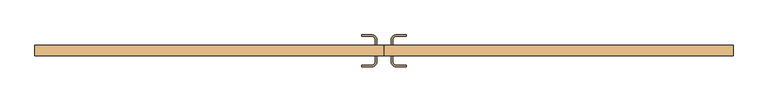
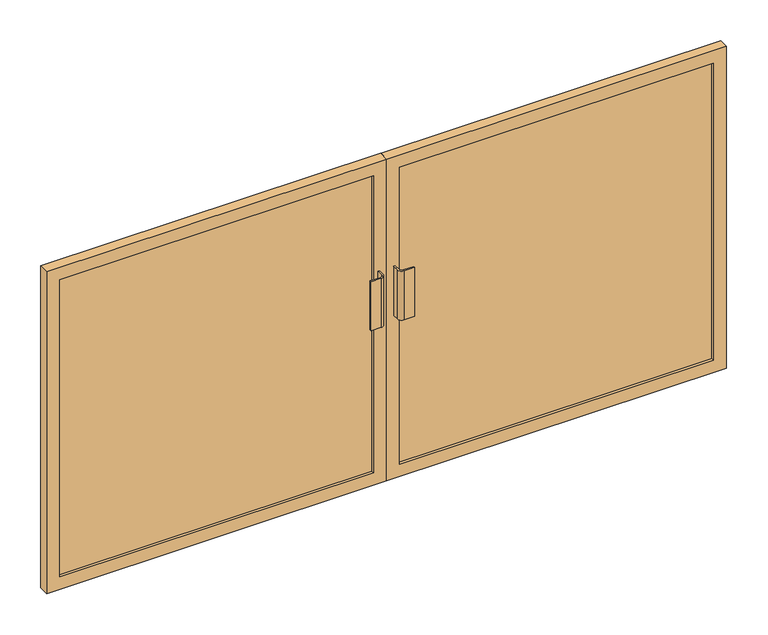
"""IFC4 building model written with IfcOpenShell, lengths in millimetres: door geometry, Porta-Parede-Cortina-Frente de loja-Dupla : Porta-Parede-Cortina-Frente de loja-Dupla."""

from ifc_helpers import new_model, si_unit, point, frame, frame_2d, origin, place, context, project, spatial, polyline, circle_curve, trimmed, segment, composite_curve, outline, extrude, source, transform, mapped, element, save


def door_319e0233(model_context):
    return source(origin(), model_context, "Body", "SweptSolid", [
        extrude(outline(polyline([(1500.0, 0.8168501), (0.0, 0.8168501), (0.0, 1500.0000075), (1500.0, 1500.0000075), (1500.0, 0.8168501)]), holes=[polyline([(1442.85, 57.9668501), (1442.85, 1442.8500075), (57.15, 1442.8500075), (57.15, 57.9668501), (1442.85, 57.9668501)])]), frame((0.0, 15.55, 0.0), z_axis=(0.0, 1.0, 0.0), x_axis=(0.0, 0.0, 1.0)), (0.0, 0.0, 1.0), 44.45),
        extrude(outline(polyline([(1500.0, -0.7706499), (1500.0, -1500.0000075), (0.0, -1500.0000075), (0.0, -0.7706499), (1500.0, -0.7706499)]), holes=[polyline([(1442.85, -1442.8500075), (1442.85, -57.9206499), (57.15, -57.9206499), (57.15, -1442.8500075), (1442.85, -1442.8500075)])]), frame((0.0, 15.55, 0.0), z_axis=(0.0, 1.0, 0.0), x_axis=(0.0, 0.0, 1.0)), (0.0, 0.0, 1.0), 44.45),
        extrude(outline(polyline([(1442.8500075, 28.25), (57.9668501, 28.25), (57.9668501, 47.3), (1442.8500075, 47.3), (1442.8500075, 28.25)])), frame((0.0, 0.0, 57.15), z_axis=(0.0, 0.0, 1.0), x_axis=(1.0, 0.0, 0.0)), (0.0, 0.0, 1.0), 1385.7),
        extrude(outline(polyline([(-57.9206499, 28.25), (-1442.8500075, 28.25), (-1442.8500075, 47.3), (-57.9206499, 47.3), (-57.9206499, 28.25)])), frame((0.0, 0.0, 57.15), z_axis=(0.0, 0.0, 1.0), x_axis=(1.0, 0.0, 0.0)), (0.0, 0.0, 1.0), 1385.7),
        extrude(outline(composite_curve([segment(trimmed(circle_curve(frame_2d((-50.7768999, -12.7)), 19.05), [point((-31.7268999, -12.7))], [point((-50.7768999, -31.75))], False, "CARTESIAN"), True, "CONTINUOUS"), segment(polyline([(-50.7768999, -31.75), (-95.2268999, -31.75), (-95.2268999, -25.4), (-50.7768999, -25.4)]), True, "CONTINUOUS"), segment(trimmed(circle_curve(frame_2d((-50.7768999, -12.7)), 12.7), [point((-50.7768999, -25.4))], [point((-38.0768999, -12.7))], True, "CARTESIAN"), True, "CONTINUOUS"), segment(polyline([(-38.0768999, -12.7), (-38.0768999, 15.55), (-31.7268999, 15.55), (-31.7268999, -12.7)]), True, "CONTINUOUS")], self_intersect=False)), frame((0.0, 0.0, 762.0), z_axis=(0.0, 0.0, 1.0), x_axis=(1.0, 0.0, 0.0)), (0.0, 0.0, 1.0), 228.6),
        extrude(outline(composite_curve([segment(polyline([(31.7731001, -12.7), (31.7731001, 15.55), (38.1231001, 15.55), (38.1231001, -12.7)]), True, "CONTINUOUS"), segment(trimmed(circle_curve(frame_2d((50.8231001, -12.7)), 12.7), [point((38.1231001, -12.7))], [point((50.8231001, -25.4))], True, "CARTESIAN"), True, "CONTINUOUS"), segment(polyline([(50.8231001, -25.4), (95.2731001, -25.4), (95.2731001, -31.75), (50.8231001, -31.75)]), True, "CONTINUOUS"), segment(trimmed(circle_curve(frame_2d((50.8231001, -12.7)), 19.05), [point((50.8231001, -31.75))], [point((31.7731001, -12.7))], False, "CARTESIAN"), True, "CONTINUOUS")], self_intersect=False)), frame((0.0, 0.0, 762.0), z_axis=(0.0, 0.0, 1.0), x_axis=(1.0, 0.0, 0.0)), (0.0, 0.0, 1.0), 228.6),
        extrude(outline(composite_curve([segment(polyline([(-31.7268999, 85.4), (-31.7268999, 60.0), (-38.0768999, 60.0), (-38.0768999, 85.4)]), True, "CONTINUOUS"), segment(trimmed(circle_curve(frame_2d((-50.7768999, 85.4)), 12.7), [point((-38.0768999, 85.4))], [point((-50.7768999, 98.1))], True, "CARTESIAN"), True, "CONTINUOUS"), segment(polyline([(-50.7768999, 98.1), (-95.2268999, 98.1), (-95.2268999, 104.45), (-50.7768999, 104.45)]), True, "CONTINUOUS"), segment(trimmed(circle_curve(frame_2d((-50.7768999, 85.4)), 19.05), [point((-50.7768999, 104.45))], [point((-31.7268999, 85.4))], False, "CARTESIAN"), True, "CONTINUOUS")], self_intersect=False)), frame((0.0, 0.0, 762.0), z_axis=(0.0, 0.0, 1.0), x_axis=(1.0, 0.0, 0.0)), (0.0, 0.0, 1.0), 228.6),
        extrude(outline(composite_curve([segment(trimmed(circle_curve(frame_2d((50.8231001, 85.4)), 19.05), [point((31.7731001, 85.4))], [point((50.8231001, 104.45))], False, "CARTESIAN"), True, "CONTINUOUS"), segment(polyline([(50.8231001, 104.45), (95.2731001, 104.45), (95.2731001, 98.1), (50.8231001, 98.1)]), True, "CONTINUOUS"), segment(trimmed(circle_curve(frame_2d((50.8231001, 85.4)), 12.7), [point((50.8231001, 98.1))], [point((38.1231001, 85.4))], True, "CARTESIAN"), True, "CONTINUOUS"), segment(polyline([(38.1231001, 85.4), (38.1231001, 60.0), (31.7731001, 60.0), (31.7731001, 85.4)]), True, "CONTINUOUS")], self_intersect=False)), frame((0.0, 0.0, 762.0), z_axis=(0.0, 0.0, 1.0), x_axis=(1.0, 0.0, 0.0)), (0.0, 0.0, 1.0), 228.6),
    ])


if __name__ == "__main__":
    model = new_model("IFC4")
    model_context = context("Model", 3, world=origin())
    ifc_project = project(units=[si_unit("LENGTHUNIT", "METRE", prefix="MILLI")], contexts=[model_context])
    site = spatial("IfcSite", under=ifc_project)
    building = spatial("IfcBuilding", under=site)
    placement = place(None, origin())
    door_shape = door_319e0233(model_context)
    element("IfcDoor", 1, ObjectType="Porta-Parede-Cortina-Frente de loja-Dupla : Porta-Parede-Cortina-Frente de loja-Dupla", at=placement, inside=building, context=model_context, shape_type="MappedRepresentation", body=[
        mapped(door_shape, transform((0.0, 0.0, 0.0), x_axis=(1.0, 0.0, 0.0), y_axis=(0.0, 1.0, 0.0), z_axis=(0.0, 0.0, 1.0))),
    ])
    save(model, "model.ifc")

# Revit data of these elements
# Type "Porta-Parede-Cortina-Frente de loja-Dupla : Porta-Parede-Cortina-Frente de loja-Dupla"
#   Type Mark = "40"
#   Construction Type Id = "opn-d46"
#   Assembly Code = "B2030100"
#   Analytic Construction = "Moldura de metal, porta de vidro duplo"
#   Largura [instance default] = 1.80 m
#   Thermal Resistance (R) = 0.242926 (m²·K)/W
#   Ângulo de abertura [instance default] = 90.00°
#   Largura do painel [instance default] = 0.90 m
#   Deslocamento = 0.06 m
#   Heat Transfer Coefficient (U) = 4.11674 W/(m²·K)
#   Function = 1
#   Material da moldura = Alumín. 1
#   Material da maçaneta = Alumín. 1
#   Vidraça = Vidro
#   Visual Light Transmittance = 0
#   Solar Heat Gain Coefficient = 0
# Element 1 (IfcDoor, "Porta-Parede-Cortina-Frente de loja-Dupla : Porta-Parede-Cortina-Frente de loja-Dupla")
#   Largura = 3.00 m
#   Largura do painel = 1.50 m
#   Materials on its faces: "Alumín. 1", "Vidro"
# Materials
#   "Alumín. 1": class "Metal", colour RGB 247 247 247, transparency 0, Description = "Alumín. 6061", Cost = 0
#   "Vidro": class "Vidro", colour RGB 0 128 192, transparency 0.9, Description = "Vidro de sílica", Cost = 0
